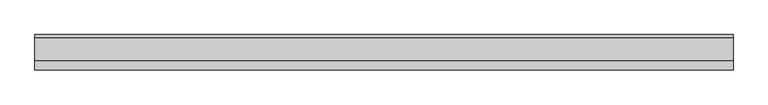
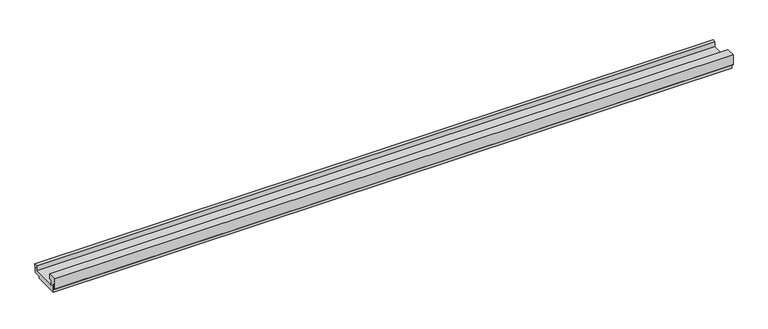
"""IFC4 building model written with IfcOpenShell, lengths in millimetres: proxy geometry, Generic Models 7:Generic Models 1:2:Generic Models 1:2 : Generic Models 7:Generic Models 1:337419:10 : Generic Models 7:Generic Models 1:2:Generic Models 1:2 : Generic Models 7:Generic Models 1:337419:306751."""

from ifc_helpers import new_model, si_unit, frame, origin, place, context, project, spatial, polyline, outline, extrude, source, transform, mapped, element, save


def generic_models_ef01e38a(model_context):
    return source(origin(), model_context, "Body", "SweptSolid", [
        extrude(outline(polyline([(-536561.6569608, 2484.834375), (-536561.6569608, 2442.765625), (-536610.8694608, 2442.765625), (-536610.8694608, 2426.890625), (-536787.8757108, 2426.890625), (-536787.8757108, 2484.834375), (-536777.9538358, 2484.834375), (-536777.9538358, 2490.7875), (-536793.8288358, 2490.7875), (-536793.8288358, 2453.293898), (-536806.9257108, 2464.2834809), (-536806.9257108, 2541.7859375), (-536741.9736944, 2541.7859375), (-536741.9736944, 2504.2140476), (-536764.0168049, 2504.2140476), (-536764.0168049, 2466.1140476), (-536579.8668049, 2466.1140476), (-536579.8668049, 2504.2140476), (-536558.8788358, 2504.2140476), (-536558.8788358, 2490.7875), (-536571.5788358, 2490.7875), (-536571.5788358, 2484.834375), (-536561.6569608, 2484.834375)])), frame((591306.0367242, 0.0, 0.0), z_axis=(1.0, 0.0, 0.0), x_axis=(0.0, 1.0, 0.0)), (0.0, 0.0, 1.0), 4876.8),
    ])


if __name__ == "__main__":
    model = new_model("IFC4")
    model_context = context("Model", 3, world=origin())
    ifc_project = project(units=[si_unit("LENGTHUNIT", "METRE", prefix="MILLI")], contexts=[model_context])
    site = spatial("IfcSite", under=ifc_project)
    building = spatial("IfcBuilding", under=site)
    placement = place(None, origin())
    generic_models_shape = generic_models_ef01e38a(model_context)
    element("IfcBuildingElementProxy", 1, Name="Generic Models 7:Generic Models 1:2:Generic Models 1:2 : Generic Models 7:Generic Models 1:337419:10 : Generic Models 7:Generic Models 1:2:Generic Models 1:2 : Generic Models 7:Generic Models 1:337419:306751", ObjectType="Generic Models 7:Generic Models 1:2:Generic Models 1:2 : Generic Models 7:Generic Models 1:337419:10 : Generic Models 7:Generic Models 1:2:Generic Models 1:2 : Generic Models 7:Generic Models 1:337419:306751", at=placement, inside=building, context=model_context, shape_type="MappedRepresentation", body=[
        mapped(generic_models_shape, transform((0.0, 0.0, 0.0), x_axis=(1.0, 0.0, 0.0), y_axis=(0.0, 1.0, 0.0), z_axis=(0.0, 0.0, 1.0))),
    ])
    save(model, "model.ifc")

# Revit data of these elements
# Type "Generic Models 7:Generic Models 1:2:Generic Models 1:2 : Generic Models 7:Generic Models 1:337419:10 : Generic Models 7:Generic Models 1:2:Generic Models 1:2 : Generic Models 7:Generic Models 1:337419:306751"
#   NameOverride = "Generic Models 7:Generic Models 1:2:Generic Models 1:2 : Generic Models 7:Generic Models 1:337419:306751"
#   ObjectTypeOverride = "Generic Models 1:2 : Generic Models 7:Generic Models 1:337419"
#   Reference = "Generic Models 1"
#   Tag = "306751"
# Element 1 (IfcBuildingElementProxy, "Generic Models 7:Generic Models 1:2:Generic Models 1:2 : Generic Models 7:Generic Models 1:337419:10 : Generic Models 7:Generic Models 1:2:Generic Models 1:2 : Generic Models 7:Generic Models 1:337419:306751")
#   Materials on its faces: "LOW VOLUMN EXPANDABLE FOAM INSULATION (CLASS A FLAME SPREAD)"
# Materials
#   "LOW VOLUMN EXPANDABLE FOAM INSULATION (CLASS A FLAME SPREAD)": class "Unassigned", colour RGB 213 216 95, transparency 0, Cost = 0
